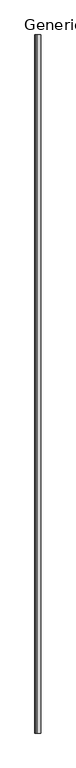
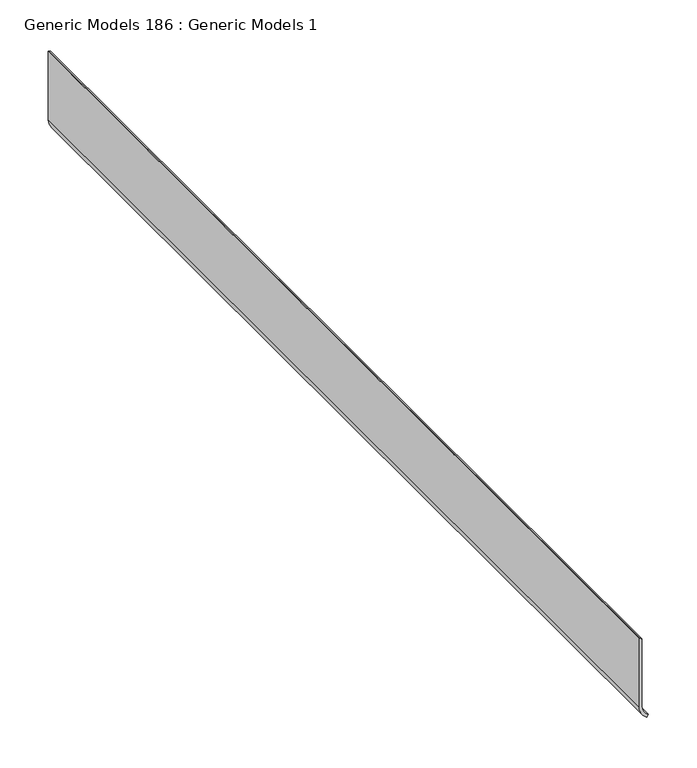
"""IFC4 building model written with IfcOpenShell, lengths in millimetres: proxy geometry, Generic Models 186 : Generic Models 1."""

from ifc_helpers import new_model, si_unit, point, frame, frame_2d, origin, place, context, project, spatial, polyline, circle_curve, trimmed, segment, composite_curve, outline, extrude, source, transform, mapped, element, save


def generic_models_186_generic_models_1_ef70466a(model_context):
    return source(origin(), model_context, "Body", "SweptSolid", [
        extrude(outline(composite_curve([segment(polyline([(101.6, 49799.875), (15.4496307, 49799.875)]), True, "CONTINUOUS"), segment(trimmed(circle_curve(frame_2d((15.4496307, 49817.7146968)), 17.8396968), [point((15.4496307, 49799.875))], [point((0.0, 49808.7948484))], False, "CARTESIAN"), True, "CONTINUOUS"), segment(polyline([(0.0, 49808.7948484), (2.7496307, 49810.3823484)]), True, "CONTINUOUS"), segment(trimmed(circle_curve(frame_2d((15.4496307, 49817.7146968)), 14.6646968), [point((2.7496307, 49810.3823484))], [point((15.4496307, 49803.05))], True, "CARTESIAN"), True, "CONTINUOUS"), segment(polyline([(15.4496307, 49803.05), (99.5131982, 49803.05)]), True, "CONTINUOUS"), segment(trimmed(circle_curve(frame_2d((99.5131982, 49800.9631982)), 2.0868018), [point((99.5131982, 49803.05))], [point((101.6, 49800.9631982))], False, "CARTESIAN"), True, "CONTINUOUS"), segment(polyline([(101.6, 49800.9631982), (101.6, 49799.875)]), True, "CONTINUOUS")], self_intersect=False)), frame((0.0, 0.0, 0.0), z_axis=(0.0, 1.0, 0.0), x_axis=(0.0, 0.0, 1.0)), (0.0, 0.0, 1.0), 1219.2),
    ])


if __name__ == "__main__":
    model = new_model("IFC4")
    model_context = context("Model", 3, world=origin())
    ifc_project = project(units=[si_unit("LENGTHUNIT", "METRE", prefix="MILLI")], contexts=[model_context])
    site = spatial("IfcSite", under=ifc_project)
    building = spatial("IfcBuilding", under=site)
    placement = place(None, origin())
    generic_models_186_generic_models_1_shape = generic_models_186_generic_models_1_ef70466a(model_context)
    element("IfcBuildingElementProxy", 1, Name="Generic Models 186 : Generic Models 1", ObjectType="Generic Models 186 : Generic Models 1", at=placement, inside=building, context=model_context, shape_type="MappedRepresentation", body=[
        mapped(generic_models_186_generic_models_1_shape, transform((0.0, 0.0, 0.0), x_axis=(1.0, 0.0, 0.0), y_axis=(0.0, 1.0, 0.0), z_axis=(0.0, 0.0, 1.0))),
    ])
    save(model, "model.ifc")

# Revit data of these elements
# Element 1 (IfcBuildingElementProxy, "Generic Models 186 : Generic Models 1")
#   Materials on its faces: "MATCH EXISTING BASE"
# Materials
#   "MATCH EXISTING BASE": class "Generic", colour RGB 120 120 120, transparency 0, Cost = 0
